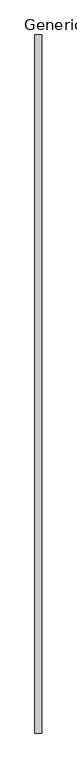
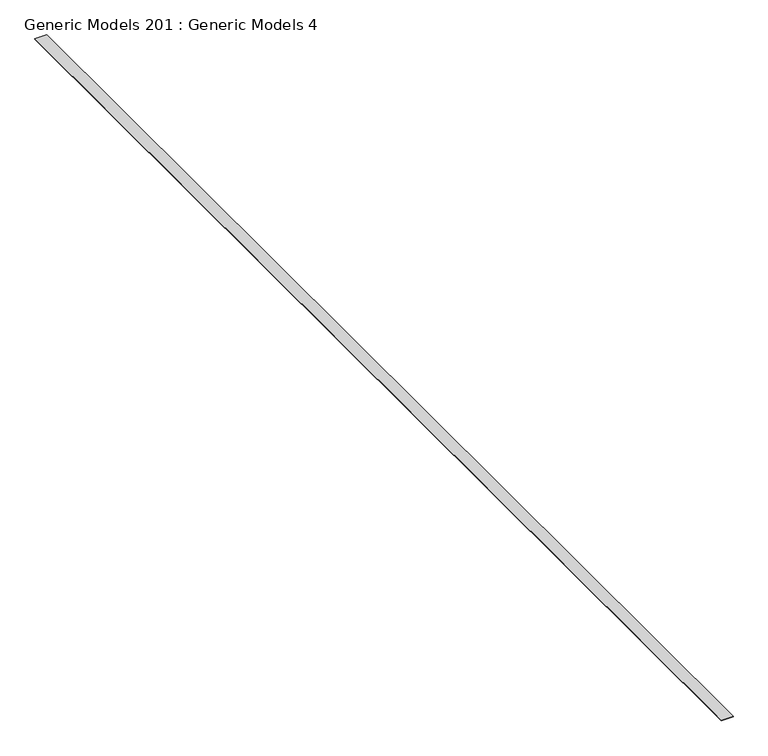
"""IFC4 building model written with IfcOpenShell, lengths in millimetres: proxy geometry, Generic Models 201 : Generic Models 4."""

from ifc_helpers import new_model, si_unit, frame, origin, place, context, project, spatial, polyline, outline, extrude, source, transform, mapped, element, save


def generic_models_201_generic_models_4_b0fb804f(model_context):
    return source(origin(), model_context, "Body", "SweptSolid", [
        extrude(outline(polyline([(-8191.6736296, -5493.3230338), (-8318.6736296, -5493.3230338), (-8318.6736296, 7054.2769662), (-8191.6736296, 7054.2769662), (-8191.6736296, -5493.3230338)])), frame((0.0, 0.0, 126790.196), z_axis=(0.0, 0.0, 1.0), x_axis=(1.0, 0.0, 0.0)), (0.0, 0.0, 1.0), 6.35),
    ])


if __name__ == "__main__":
    model = new_model("IFC4")
    model_context = context("Model", 3, world=origin())
    ifc_project = project(units=[si_unit("LENGTHUNIT", "METRE", prefix="MILLI")], contexts=[model_context])
    site = spatial("IfcSite", under=ifc_project)
    building = spatial("IfcBuilding", under=site)
    placement = place(None, origin())
    generic_models_201_generic_models_4_shape = generic_models_201_generic_models_4_b0fb804f(model_context)
    element("IfcBuildingElementProxy", 1, Name="Generic Models 201 : Generic Models 4", ObjectType="Generic Models 201 : Generic Models 4", at=placement, inside=building, context=model_context, shape_type="MappedRepresentation", body=[
        mapped(generic_models_201_generic_models_4_shape, transform((0.0, 0.0, 0.0), x_axis=(1.0, 0.0, 0.0), y_axis=(0.0, 1.0, 0.0), z_axis=(0.0, 0.0, 1.0))),
    ])
    save(model, "model.ifc")

# Revit data of these elements
# Element 1 (IfcBuildingElementProxy, "Generic Models 201 : Generic Models 4")
#   Materials on its faces: "_STEEL BASE PLATE AT EACH RAILING POST (SEE STRUCT. DWGS)"
# Materials
#   "_STEEL BASE PLATE AT EACH RAILING POST (SEE STRUCT. DWGS)": class "Generic", colour RGB 233 233 233, transparency 0, Cost = 0
